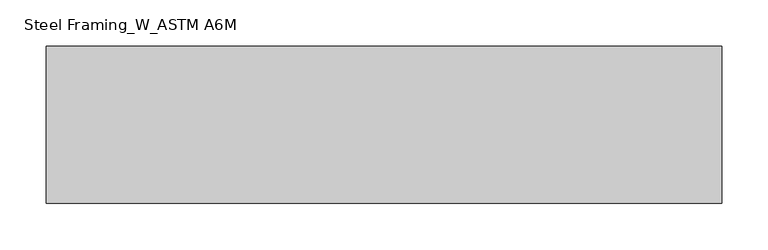
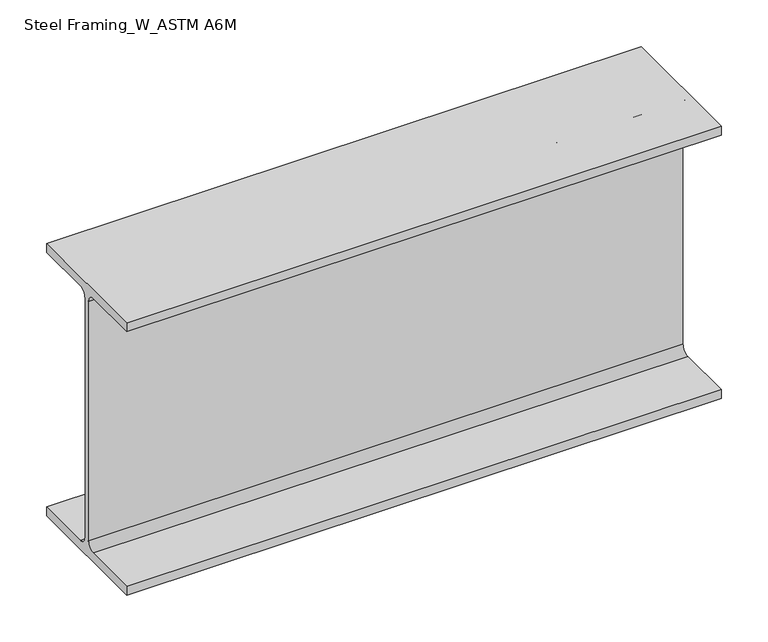
"""IFC4 building model written with IfcOpenShell, lengths in millimetres: beam geometry, Steel Framing_W_ASTM A6M : H_SB_AR_S02_W360x51_RG1."""

from ifc_helpers import new_model, si_unit, point, frame, frame_2d, origin, place, context, project, spatial, polyline, circle_curve, trimmed, segment, composite_curve, outline, extrude, source, transform, mapped, element, save


def steel_framing_w_astm_a6m_e9389756(model_context):
    return source(origin(), model_context, "Body", "SweptSolid", [
        extrude(outline(composite_curve([segment(polyline([(85.5, -166.4), (85.5, -178.0), (-85.5, -178.0), (-85.5, -166.4), (-13.72, -166.4)]), True, "CONTINUOUS"), segment(trimmed(circle_curve(frame_2d((-13.72, -156.3)), 10.1), [point((-13.72, -166.4))], [point((-3.62, -156.3))], True, "CARTESIAN"), True, "CONTINUOUS"), segment(polyline([(-3.62, -156.3), (-3.62, 156.3)]), True, "CONTINUOUS"), segment(trimmed(circle_curve(frame_2d((-13.72, 156.3)), 10.1), [point((-3.62, 156.3))], [point((-13.72, 166.4))], True, "CARTESIAN"), True, "CONTINUOUS"), segment(polyline([(-13.72, 166.4), (-85.5, 166.4), (-85.5, 178.0), (85.5, 178.0), (85.5, 166.4), (13.72, 166.4)]), True, "CONTINUOUS"), segment(trimmed(circle_curve(frame_2d((13.72, 156.3)), 10.1), [point((13.72, 166.4))], [point((3.62, 156.3))], True, "CARTESIAN"), True, "CONTINUOUS"), segment(polyline([(3.62, 156.3), (3.62, -156.3)]), True, "CONTINUOUS"), segment(trimmed(circle_curve(frame_2d((13.72, -156.3)), 10.1), [point((3.62, -156.3))], [point((13.72, -166.4))], True, "CARTESIAN"), True, "CONTINUOUS"), segment(polyline([(13.72, -166.4), (85.5, -166.4)]), True, "CONTINUOUS")], self_intersect=False)), frame((-211.15, 0.0, 0.0), z_axis=(1.0, 0.0, 0.0), x_axis=(0.0, 1.0, 0.0)), (0.0, 0.0, 1.0), 734.3),
    ])


if __name__ == "__main__":
    model = new_model("IFC4")
    model_context = context("Model", 3, world=origin())
    ifc_project = project(units=[si_unit("LENGTHUNIT", "METRE", prefix="MILLI")], contexts=[model_context])
    site = spatial("IfcSite", under=ifc_project)
    building = spatial("IfcBuilding", under=site)
    placement = place(None, origin())
    steel_framing_w_astm_a6m_shape = steel_framing_w_astm_a6m_e9389756(model_context)
    element("IfcBeam", 1, ObjectType="Steel Framing_W_ASTM A6M : H_SB_AR_S02_W360x51_RG1", at=placement, inside=building, context=model_context, shape_type="MappedRepresentation", body=[
        mapped(steel_framing_w_astm_a6m_shape, transform((0.0, 0.0, 0.0), x_axis=(1.0, 0.0, 0.0), y_axis=(0.0, 1.0, 0.0), z_axis=(0.0, 0.0, 1.0))),
    ])
    save(model, "model.ifc")

# Revit data of these elements
# Type "Steel Framing_W_ASTM A6M : H_SB_AR_S02_W360x51_RG1"
#   Type Mark = "RG1"
#   Section Name Key = "W14x34"
#   Width = 17.1 cm
#   Web Thickness = 0.724 cm
#   Web Fillet = 1.01 cm
#   Warping Constant = 287000.0 cm⁶
#   Torsional Moment of Inertia = 23.70 cm⁴
#   Section Area = 64.5 cm²
#   Plastic Modulus weak axis = 174.0 cm³
#   Plastic Modulus strong axis = 895.0 cm³
#   Perimeter = 1.36 m²/m
#   Nominal Weight = 51.00 kgf/m
#   Moment of Inertia weak axis = 970.00 cm⁴
#   Moment of Inertia strong axis = 14200.00 cm⁴
#   Height = 35.6 cm
#   Flange Thickness = 1.16 cm
#   Elastic Modulus weak axis = 113.0 cm³
#   Elastic Modulus strong axis = 796.0 cm³
#   Centroid Vertical = 17.8 cm
#   Centroid Horizontal = 8.55 cm
#   Length [instance default] = 1500 mm
#   Structural Material [instance default] = Steel, 45-345
#   Bolt Spacing = 0
#   Assembly Code = ""
# Element 1 (IfcBeam, "Steel Framing_W_ASTM A6M : H_SB_AR_S02_W360x51_RG1")
#   Materials on its faces: "Steel, 45-345"
# Materials
#   "Steel, 45-345": class "Metal", colour RGB 189 187 185, transparency 0, Description = "Steel 345 MPa", Cost = 0
